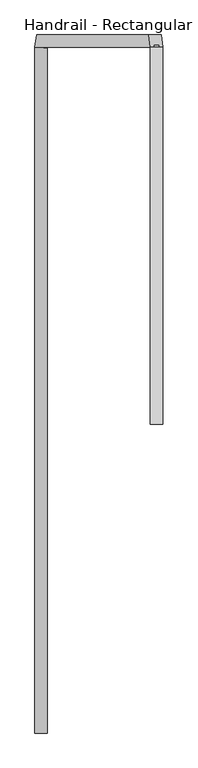
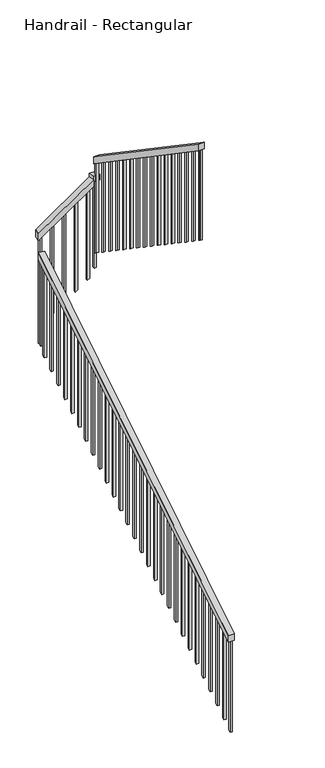
"""IFC4 building model written with IfcOpenShell, lengths in millimetres: railing geometry, Handrail - Rectangular."""

from ifc_helpers import new_model, si_unit, frame, origin, place, context, project, spatial, polyline, outline, extrude, faceted_brep, source, transform, mapped, element, save


def handrail_rectangular_e170ce91(model_context):
    return source(origin(), model_context, "Body", "SolidModel", [
        faceted_brep([(-4295.7586735, -1605.5757069, -2569.0285714), (-4346.5586735, -1605.5757069, -2569.0285714), (-4346.5586735, -1605.5757069, -2628.8906848), (-4295.7586735, -1605.5757069, -2628.8906848), (-4295.7586735, 1183.5282571, -830.3663601), (-4295.7586735, 1183.5282571, -890.2284734), (-4346.5586735, 1190.0652515, -886.1534639), (-4346.5586735, 1190.0652515, -826.2913506)], [[[0, 1, 2, 3]], [[4, 5, 6, 7]], [[1, 0, 4, 7]], [[2, 1, 7, 6]], [[3, 2, 6, 5]], [[0, 3, 5, 4]]]),
        faceted_brep([(-4346.7456679, 1186.9711303, -657.6253676), (-4340.2086735, 1237.7711303, -653.1428571), (-4340.2086735, 1237.7711303, -714.7388591), (-4346.7456679, 1186.9711303, -719.2213696), (-3876.8905457, 1186.9711303, -335.4389981), (-3876.8905457, 1186.9711303, -397.0350001), (-3883.4275401, 1237.7711303, -401.5175105), (-3883.4275401, 1237.7711303, -339.9215085)], [[[0, 1, 2, 3]], [[4, 5, 6, 7]], [[1, 0, 4, 7]], [[2, 1, 7, 6]], [[3, 2, 6, 5]], [[0, 3, 5, 4]]]),
        faceted_brep([(-3883.4275401, 1237.7711303, -304.8), (-3832.2086735, 1237.7711303, -304.8), (-3832.2086735, 1237.7711303, -355.6), (-3883.4275401, 1237.7711303, -355.6), (-3876.8681068, 1186.7967543, -304.8), (-3876.8681068, 1186.7967543, -355.6), (-3825.6492402, 1186.7967543, -355.6), (-3825.6492402, 1186.7967543, -304.8)], [[[0, 1, 2, 3]], [[4, 5, 6, 7]], [[1, 0, 4, 7]], [[2, 1, 7, 6]], [[3, 2, 6, 5]], [[0, 3, 5, 4]]]),
        faceted_brep([(-3876.6586735, 1186.7967543, -129.5217682), (-3825.8586735, 1186.7967543, -129.5217682), (-3825.8586735, 1186.7967543, -190.9554209), (-3876.6586735, 1186.7967543, -190.9554209), (-3876.6586735, -348.2757069, 914.4), (-3876.6586735, -348.2757069, 852.9663473), (-3825.8586735, -348.2757069, 852.9663473), (-3825.8586735, -348.2757069, 914.4)], [[[0, 1, 2, 3]], [[4, 5, 6, 7]], [[1, 0, 4, 7]], [[2, 1, 7, 6]], [[3, 2, 6, 5]], [[0, 3, 5, 4]]]),
        extrude(outline(polyline([(-346.7282457, 851.9140005), (-327.6782457, 838.9591009), (-327.6782457, 31.2396761), (-346.7282457, 44.1945758), (-346.7282457, 851.9140005)])), frame((-3860.7836735, 0.0, 0.0), z_axis=(1.0, 0.0, 0.0), x_axis=(0.0, 1.0, 0.0)), (0.0, 0.0, 1.0), 19.05),
        extrude(outline(polyline([(-245.1282457, 782.8212024), (-226.0782457, 769.8663028), (-226.0782457, -37.853122), (-245.1282457, -24.8982224), (-245.1282457, 782.8212024)])), frame((-3860.7836735, 0.0, 0.0), z_axis=(1.0, 0.0, 0.0), x_axis=(0.0, 1.0, 0.0)), (0.0, 0.0, 1.0), 19.05),
        extrude(outline(polyline([(-143.5282457, 713.7284043), (-124.4782457, 700.7735047), (-124.4782457, -106.9459201), (-143.5282457, -93.9910205), (-143.5282457, 713.7284043)])), frame((-3860.7836735, 0.0, 0.0), z_axis=(1.0, 0.0, 0.0), x_axis=(0.0, 1.0, 0.0)), (0.0, 0.0, 1.0), 19.05),
        extrude(outline(polyline([(-41.9282457, 644.6356062), (-22.8782457, 631.6807066), (-22.8782457, -176.0387182), (-41.9282457, -163.0838186), (-41.9282457, 644.6356062)])), frame((-3860.7836735, 0.0, 0.0), z_axis=(1.0, 0.0, 0.0), x_axis=(0.0, 1.0, 0.0)), (0.0, 0.0, 1.0), 19.05),
        extrude(outline(polyline([(59.6717543, 575.5428081), (78.7217543, 562.5879084), (78.7217543, -245.1315163), (59.6717543, -232.1766167), (59.6717543, 575.5428081)])), frame((-3860.7836735, 0.0, 0.0), z_axis=(1.0, 0.0, 0.0), x_axis=(0.0, 1.0, 0.0)), (0.0, 0.0, 1.0), 19.05),
        extrude(outline(polyline([(161.2717543, 506.45001), (180.3217543, 493.4951103), (180.3217543, -314.2243144), (161.2717543, -301.2694148), (161.2717543, 506.45001)])), frame((-3860.7836735, 0.0, 0.0), z_axis=(1.0, 0.0, 0.0), x_axis=(0.0, 1.0, 0.0)), (0.0, 0.0, 1.0), 19.05),
        extrude(outline(polyline([(262.8717543, 437.3572119), (281.9217543, 424.4023122), (281.9217543, -383.3171126), (262.8717543, -370.3622129), (262.8717543, 437.3572119)])), frame((-3860.7836735, 0.0, 0.0), z_axis=(1.0, 0.0, 0.0), x_axis=(0.0, 1.0, 0.0)), (0.0, 0.0, 1.0), 19.05),
        extrude(outline(polyline([(364.4717543, 368.2644138), (383.5217543, 355.3095141), (383.5217543, -452.4099107), (364.4717543, -439.455011), (364.4717543, 368.2644138)])), frame((-3860.7836735, 0.0, 0.0), z_axis=(1.0, 0.0, 0.0), x_axis=(0.0, 1.0, 0.0)), (0.0, 0.0, 1.0), 19.05),
        extrude(outline(polyline([(466.0717543, 299.1716157), (485.1217543, 286.216716), (485.1217543, -521.5027088), (466.0717543, -508.5478091), (466.0717543, 299.1716157)])), frame((-3860.7836735, 0.0, 0.0), z_axis=(1.0, 0.0, 0.0), x_axis=(0.0, 1.0, 0.0)), (0.0, 0.0, 1.0), 19.05),
        extrude(outline(polyline([(567.6717543, 230.0788175), (586.7217543, 217.1239179), (586.7217543, -590.5955069), (567.6717543, -577.6406072), (567.6717543, 230.0788175)])), frame((-3860.7836735, 0.0, 0.0), z_axis=(1.0, 0.0, 0.0), x_axis=(0.0, 1.0, 0.0)), (0.0, 0.0, 1.0), 19.05),
        extrude(outline(polyline([(669.2717543, 160.9860194), (688.3217543, 148.0311198), (688.3217543, -659.688305), (669.2717543, -646.7334054), (669.2717543, 160.9860194)])), frame((-3860.7836735, 0.0, 0.0), z_axis=(1.0, 0.0, 0.0), x_axis=(0.0, 1.0, 0.0)), (0.0, 0.0, 1.0), 19.05),
        extrude(outline(polyline([(770.8717543, 91.8932213), (789.9217543, 78.9383217), (789.9217543, -728.7811031), (770.8717543, -715.8262035), (770.8717543, 91.8932213)])), frame((-3860.7836735, 0.0, 0.0), z_axis=(1.0, 0.0, 0.0), x_axis=(0.0, 1.0, 0.0)), (0.0, 0.0, 1.0), 19.05),
        extrude(outline(polyline([(872.4717543, 22.8004232), (891.5217543, 9.8455236), (891.5217543, -797.8739012), (872.4717543, -784.9190016), (872.4717543, 22.8004232)])), frame((-3860.7836735, 0.0, 0.0), z_axis=(1.0, 0.0, 0.0), x_axis=(0.0, 1.0, 0.0)), (0.0, 0.0, 1.0), 19.05),
        extrude(outline(polyline([(974.0717543, -46.2923749), (993.1217543, -59.2472745), (993.1217543, -866.9666993), (974.0717543, -854.0117997), (974.0717543, -46.2923749)])), frame((-3860.7836735, 0.0, 0.0), z_axis=(1.0, 0.0, 0.0), x_axis=(0.0, 1.0, 0.0)), (0.0, 0.0, 1.0), 19.05),
        extrude(outline(polyline([(1075.6717543, -115.385173), (1094.7217543, -128.3400727), (1094.7217543, -936.0594974), (1075.6717543, -923.1045978), (1075.6717543, -115.385173)])), frame((-3860.7836735, 0.0, 0.0), z_axis=(1.0, 0.0, 0.0), x_axis=(0.0, 1.0, 0.0)), (0.0, 0.0, 1.0), 19.05),
        extrude(outline(polyline([(-414.2136458, -3901.9427374), (-427.276503, -3920.9927374), (-1234.2423487, -3920.9927374), (-1221.1794915, -3901.9427374), (-414.2136458, -3901.9427374)])), frame((0.0, 1202.8461303, 0.0), z_axis=(0.0, 1.0, 0.0), x_axis=(0.0, 0.0, 1.0)), (0.0, 0.0, 1.0), 19.05),
        extrude(outline(polyline([(-483.8822172, -4003.5427374), (-496.9450744, -4022.5927374), (-1303.9109201, -4022.5927374), (-1290.8480629, -4003.5427374), (-483.8822172, -4003.5427374)])), frame((0.0, 1202.8461303, 0.0), z_axis=(0.0, 1.0, 0.0), x_axis=(0.0, 0.0, 1.0)), (0.0, 0.0, 1.0), 19.05),
        extrude(outline(polyline([(-553.5507887, -4105.1427374), (-566.6136458, -4124.1927374), (-1373.5794915, -4124.1927374), (-1360.5166344, -4105.1427374), (-553.5507887, -4105.1427374)])), frame((0.0, 1202.8461303, 0.0), z_axis=(0.0, 1.0, 0.0), x_axis=(0.0, 0.0, 1.0)), (0.0, 0.0, 1.0), 19.05),
        extrude(outline(polyline([(-623.2193601, -4206.7427374), (-636.2822172, -4225.7927374), (-1443.2480629, -4225.7927374), (-1430.1852058, -4206.7427374), (-623.2193601, -4206.7427374)])), frame((0.0, 1202.8461303, 0.0), z_axis=(0.0, 1.0, 0.0), x_axis=(0.0, 0.0, 1.0)), (0.0, 0.0, 1.0), 19.05),
        extrude(outline(polyline([(1128.0992931, -924.7815939), (1147.1492931, -912.9062692), (1147.1492931, -1727.8627539), (1128.0992931, -1739.7380786), (1128.0992931, -924.7815939)])), frame((-4330.6836735, 0.0, 0.0), z_axis=(1.0, 0.0, 0.0), x_axis=(0.0, 1.0, 0.0)), (0.0, 0.0, 1.0), 19.05),
        extrude(outline(polyline([(1026.4992931, -988.1166588), (1045.5492931, -976.2413341), (1045.5492931, -1791.1978188), (1026.4992931, -1803.0731435), (1026.4992931, -988.1166588)])), frame((-4330.6836735, 0.0, 0.0), z_axis=(1.0, 0.0, 0.0), x_axis=(0.0, 1.0, 0.0)), (0.0, 0.0, 1.0), 19.05),
        extrude(outline(polyline([(924.8992931, -1051.4517237), (943.9492931, -1039.576399), (943.9492931, -1854.5328838), (924.8992931, -1866.4082084), (924.8992931, -1051.4517237)])), frame((-4330.6836735, 0.0, 0.0), z_axis=(1.0, 0.0, 0.0), x_axis=(0.0, 1.0, 0.0)), (0.0, 0.0, 1.0), 19.05),
        extrude(outline(polyline([(823.2992931, -1114.7867887), (842.3492931, -1102.911464), (842.3492931, -1917.8679487), (823.2992931, -1929.7432734), (823.2992931, -1114.7867887)])), frame((-4330.6836735, 0.0, 0.0), z_axis=(1.0, 0.0, 0.0), x_axis=(0.0, 1.0, 0.0)), (0.0, 0.0, 1.0), 19.05),
        extrude(outline(polyline([(721.6992931, -1178.1218536), (740.7492931, -1166.2465289), (740.7492931, -1981.2030136), (721.6992931, -1993.0783383), (721.6992931, -1178.1218536)])), frame((-4330.6836735, 0.0, 0.0), z_axis=(1.0, 0.0, 0.0), x_axis=(0.0, 1.0, 0.0)), (0.0, 0.0, 1.0), 19.05),
        extrude(outline(polyline([(620.0992931, -1241.4569185), (639.1492931, -1229.5815939), (639.1492931, -2044.5380786), (620.0992931, -2056.4134032), (620.0992931, -1241.4569185)])), frame((-4330.6836735, 0.0, 0.0), z_axis=(1.0, 0.0, 0.0), x_axis=(0.0, 1.0, 0.0)), (0.0, 0.0, 1.0), 19.05),
        extrude(outline(polyline([(518.4992931, -1304.7919835), (537.5492931, -1292.9166588), (537.5492931, -2107.8731435), (518.4992931, -2119.7484682), (518.4992931, -1304.7919835)])), frame((-4330.6836735, 0.0, 0.0), z_axis=(1.0, 0.0, 0.0), x_axis=(0.0, 1.0, 0.0)), (0.0, 0.0, 1.0), 19.05),
        extrude(outline(polyline([(416.8992931, -1368.1270484), (435.9492931, -1356.2517237), (435.9492931, -2171.2082084), (416.8992931, -2183.0835331), (416.8992931, -1368.1270484)])), frame((-4330.6836735, 0.0, 0.0), z_axis=(1.0, 0.0, 0.0), x_axis=(0.0, 1.0, 0.0)), (0.0, 0.0, 1.0), 19.05),
        extrude(outline(polyline([(315.2992931, -1431.4621133), (334.3492931, -1419.5867887), (334.3492931, -2234.5432734), (315.2992931, -2246.418598), (315.2992931, -1431.4621133)])), frame((-4330.6836735, 0.0, 0.0), z_axis=(1.0, 0.0, 0.0), x_axis=(0.0, 1.0, 0.0)), (0.0, 0.0, 1.0), 19.05),
        extrude(outline(polyline([(213.6992931, -1494.7971783), (232.7492931, -1482.9218536), (232.7492931, -2297.8783383), (213.6992931, -2309.753663), (213.6992931, -1494.7971783)])), frame((-4330.6836735, 0.0, 0.0), z_axis=(1.0, 0.0, 0.0), x_axis=(0.0, 1.0, 0.0)), (0.0, 0.0, 1.0), 19.05),
        extrude(outline(polyline([(112.0992931, -1558.1322432), (131.1492931, -1546.2569185), (131.1492931, -2361.2134032), (112.0992931, -2373.0887279), (112.0992931, -1558.1322432)])), frame((-4330.6836735, 0.0, 0.0), z_axis=(1.0, 0.0, 0.0), x_axis=(0.0, 1.0, 0.0)), (0.0, 0.0, 1.0), 19.05),
        extrude(outline(polyline([(10.4992931, -1621.4673081), (29.5492931, -1609.5919835), (29.5492931, -2424.5484682), (10.4992931, -2436.4237928), (10.4992931, -1621.4673081)])), frame((-4330.6836735, 0.0, 0.0), z_axis=(1.0, 0.0, 0.0), x_axis=(0.0, 1.0, 0.0)), (0.0, 0.0, 1.0), 19.05),
        extrude(outline(polyline([(-91.1007069, -1684.8023731), (-72.0507069, -1672.9270484), (-72.0507069, -2487.8835331), (-91.1007069, -2499.7588578), (-91.1007069, -1684.8023731)])), frame((-4330.6836735, 0.0, 0.0), z_axis=(1.0, 0.0, 0.0), x_axis=(0.0, 1.0, 0.0)), (0.0, 0.0, 1.0), 19.05),
        extrude(outline(polyline([(-192.7007069, -1748.137438), (-173.6507069, -1736.2621133), (-173.6507069, -2551.218598), (-192.7007069, -2563.0939227), (-192.7007069, -1748.137438)])), frame((-4330.6836735, 0.0, 0.0), z_axis=(1.0, 0.0, 0.0), x_axis=(0.0, 1.0, 0.0)), (0.0, 0.0, 1.0), 19.05),
        extrude(outline(polyline([(-294.3007069, -1811.4725029), (-275.2507069, -1799.5971783), (-275.2507069, -2614.553663), (-294.3007069, -2626.4289876), (-294.3007069, -1811.4725029)])), frame((-4330.6836735, 0.0, 0.0), z_axis=(1.0, 0.0, 0.0), x_axis=(0.0, 1.0, 0.0)), (0.0, 0.0, 1.0), 19.05),
        extrude(outline(polyline([(-395.9007069, -1874.8075679), (-376.8507069, -1862.9322432), (-376.8507069, -2677.8887279), (-395.9007069, -2689.7640526), (-395.9007069, -1874.8075679)])), frame((-4330.6836735, 0.0, 0.0), z_axis=(1.0, 0.0, 0.0), x_axis=(0.0, 1.0, 0.0)), (0.0, 0.0, 1.0), 19.05),
        extrude(outline(polyline([(-497.5007069, -1938.1426328), (-478.4507069, -1926.2673081), (-478.4507069, -2741.2237928), (-497.5007069, -2753.0991175), (-497.5007069, -1938.1426328)])), frame((-4330.6836735, 0.0, 0.0), z_axis=(1.0, 0.0, 0.0), x_axis=(0.0, 1.0, 0.0)), (0.0, 0.0, 1.0), 19.05),
        extrude(outline(polyline([(-599.1007069, -2001.4776977), (-580.0507069, -1989.6023731), (-580.0507069, -2804.5588578), (-599.1007069, -2816.4341825), (-599.1007069, -2001.4776977)])), frame((-4330.6836735, 0.0, 0.0), z_axis=(1.0, 0.0, 0.0), x_axis=(0.0, 1.0, 0.0)), (0.0, 0.0, 1.0), 19.05),
        extrude(outline(polyline([(-700.7007069, -2064.8127627), (-681.6507069, -2052.937438), (-681.6507069, -2867.8939227), (-700.7007069, -2879.7692474), (-700.7007069, -2064.8127627)])), frame((-4330.6836735, 0.0, 0.0), z_axis=(1.0, 0.0, 0.0), x_axis=(0.0, 1.0, 0.0)), (0.0, 0.0, 1.0), 19.05),
        extrude(outline(polyline([(-802.3007069, -2128.1478276), (-783.2507069, -2116.2725029), (-783.2507069, -2931.2289876), (-802.3007069, -2943.1043123), (-802.3007069, -2128.1478276)])), frame((-4330.6836735, 0.0, 0.0), z_axis=(1.0, 0.0, 0.0), x_axis=(0.0, 1.0, 0.0)), (0.0, 0.0, 1.0), 19.05),
        extrude(outline(polyline([(-903.9007069, -2191.4828926), (-884.8507069, -2179.6075679), (-884.8507069, -2994.5640526), (-903.9007069, -3006.4393773), (-903.9007069, -2191.4828926)])), frame((-4330.6836735, 0.0, 0.0), z_axis=(1.0, 0.0, 0.0), x_axis=(0.0, 1.0, 0.0)), (0.0, 0.0, 1.0), 19.05),
        extrude(outline(polyline([(-1005.5007069, -2254.8179575), (-986.4507069, -2242.9426328), (-986.4507069, -3057.8991175), (-1005.5007069, -3069.7744422), (-1005.5007069, -2254.8179575)])), frame((-4330.6836735, 0.0, 0.0), z_axis=(1.0, 0.0, 0.0), x_axis=(0.0, 1.0, 0.0)), (0.0, 0.0, 1.0), 19.05),
        extrude(outline(polyline([(-1107.1007069, -2318.1530224), (-1088.0507069, -2306.2776977), (-1088.0507069, -3121.2341825), (-1107.1007069, -3133.1095071), (-1107.1007069, -2318.1530224)])), frame((-4330.6836735, 0.0, 0.0), z_axis=(1.0, 0.0, 0.0), x_axis=(0.0, 1.0, 0.0)), (0.0, 0.0, 1.0), 19.05),
        extrude(outline(polyline([(-1208.7007069, -2381.4880874), (-1189.6507069, -2369.6127627), (-1189.6507069, -3184.5692474), (-1208.7007069, -3196.4445721), (-1208.7007069, -2381.4880874)])), frame((-4330.6836735, 0.0, 0.0), z_axis=(1.0, 0.0, 0.0), x_axis=(0.0, 1.0, 0.0)), (0.0, 0.0, 1.0), 19.05),
        extrude(outline(polyline([(-1310.3007069, -2444.8231523), (-1291.2507069, -2432.9478276), (-1291.2507069, -3247.9043123), (-1310.3007069, -3259.779637), (-1310.3007069, -2444.8231523)])), frame((-4330.6836735, 0.0, 0.0), z_axis=(1.0, 0.0, 0.0), x_axis=(0.0, 1.0, 0.0)), (0.0, 0.0, 1.0), 19.05),
        extrude(outline(polyline([(-1411.9007069, -2508.1582172), (-1392.8507069, -2496.2828926), (-1392.8507069, -3311.2393773), (-1411.9007069, -3323.1147019), (-1411.9007069, -2508.1582172)])), frame((-4330.6836735, 0.0, 0.0), z_axis=(1.0, 0.0, 0.0), x_axis=(0.0, 1.0, 0.0)), (0.0, 0.0, 1.0), 19.05),
        extrude(outline(polyline([(-1513.5007069, -2571.4932822), (-1494.4507069, -2559.6179575), (-1494.4507069, -3374.5744422), (-1513.5007069, -3386.4497669), (-1513.5007069, -2571.4932822)])), frame((-4330.6836735, 0.0, 0.0), z_axis=(1.0, 0.0, 0.0), x_axis=(0.0, 1.0, 0.0)), (0.0, 0.0, 1.0), 19.05),
        extrude(outline(polyline([(1177.2717543, -184.4779711), (1196.3217543, -197.4328708), (1196.3217543, -1005.1522956), (1177.2717543, -992.1973959), (1177.2717543, -184.4779711)])), frame((-3860.7836735, 0.0, 0.0), z_axis=(1.0, 0.0, 0.0), x_axis=(0.0, 1.0, 0.0)), (0.0, 0.0, 1.0), 19.05),
        extrude(outline(polyline([(-3865.2123772, 1220.6025723), (-3846.3181676, 1223.0338979), (-3843.886842, 1204.1396883), (-3862.7810516, 1201.7083627), (-3865.2123772, 1220.6025723)])), frame((0.0, 0.0, -1143.0), z_axis=(0.0, 0.0, 1.0), x_axis=(1.0, 0.0, 0.0)), (0.0, 0.0, 1.0), 787.4),
        extrude(outline(polyline([(-692.8879315, -4308.3427374), (-705.9507887, -4327.3927374), (-1665.5142857, -4327.3927374), (-1665.5142857, -4308.3427374), (-692.8879315, -4308.3427374)])), frame((0.0, 1202.8461303, 0.0), z_axis=(0.0, 1.0, 0.0), x_axis=(0.0, 0.0, 1.0)), (0.0, 0.0, 1.0), 19.05),
        extrude(outline(polyline([(-4312.9272315, 1176.1339867), (-4331.8214411, 1178.5653123), (-4329.3901155, 1197.4595219), (-4310.4959059, 1195.0281963), (-4312.9272315, 1176.1339867)])), frame((0.0, 0.0, -1665.5142857), z_axis=(0.0, 0.0, 1.0), x_axis=(1.0, 0.0, 0.0)), (0.0, 0.0, 1.0), 787.4),
        extrude(outline(polyline([(-348.2757069, 852.9663473), (-329.2257069, 840.0114476), (-329.2257069, 32.2920228), (-348.2757069, 45.2469225), (-348.2757069, 852.9663473)])), frame((-3860.7836735, 0.0, 0.0), z_axis=(1.0, 0.0, 0.0), x_axis=(0.0, 1.0, 0.0)), (0.0, 0.0, 1.0), 19.05),
        extrude(outline(polyline([(-1605.5757069, -2628.8906848), (-1586.5257069, -2617.0153601), (-1586.5257069, -3431.9718448), (-1605.5757069, -3443.8471695), (-1605.5757069, -2628.8906848)])), frame((-4330.6836735, 0.0, 0.0), z_axis=(1.0, 0.0, 0.0), x_axis=(0.0, 1.0, 0.0)), (0.0, 0.0, 1.0), 19.05),
    ])


if __name__ == "__main__":
    model = new_model("IFC4")
    model_context = context("Model", 3, world=origin())
    ifc_project = project(units=[si_unit("LENGTHUNIT", "METRE", prefix="MILLI")], contexts=[model_context])
    site = spatial("IfcSite", under=ifc_project)
    building = spatial("IfcBuilding", under=site)
    placement = place(None, origin())
    handrail_rectangular_shape = handrail_rectangular_e170ce91(model_context)
    element("IfcRailing", 1, ObjectType="Handrail - Rectangular", at=placement, inside=building, context=model_context, shape_type="MappedRepresentation", body=[
        mapped(handrail_rectangular_shape, transform((0.0, 0.0, 0.0), x_axis=(1.0, 0.0, 0.0), y_axis=(0.0, 1.0, 0.0), z_axis=(0.0, 0.0, 1.0))),
    ])
    save(model, "model.ifc")
